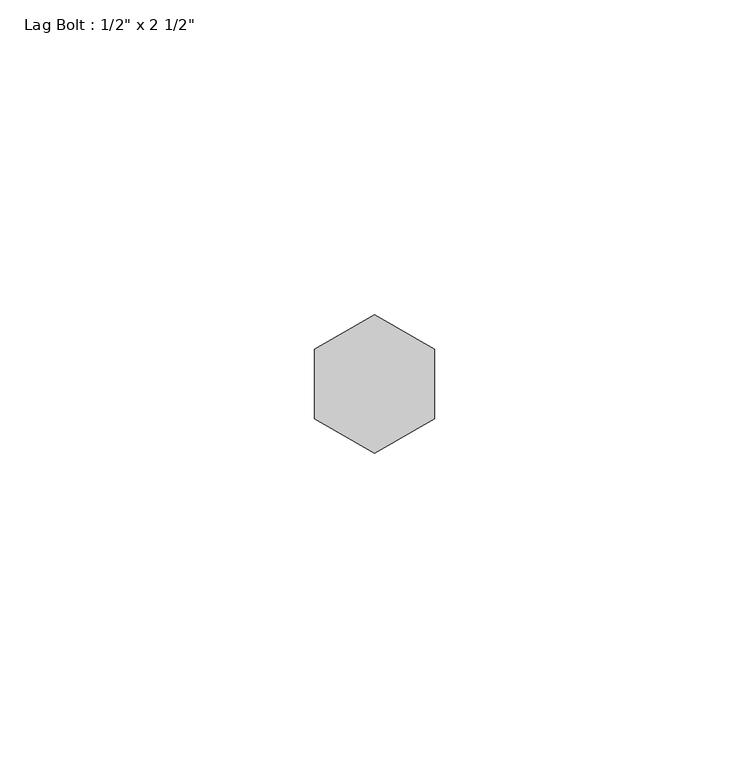
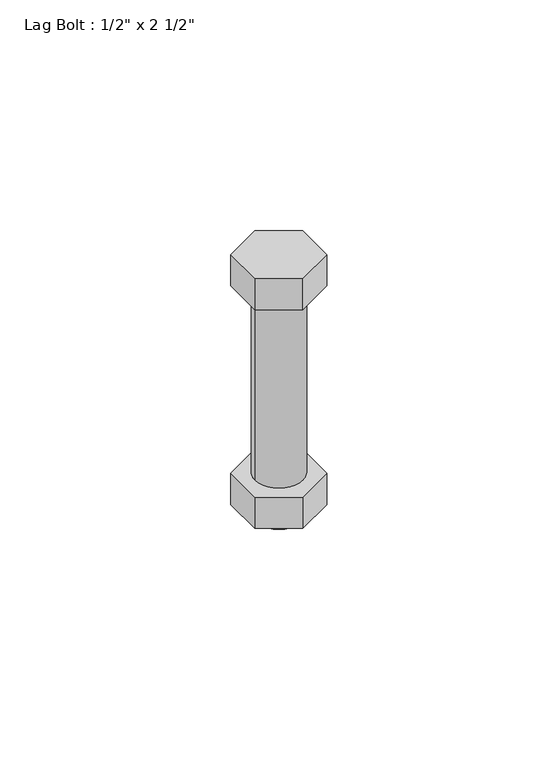
"""IFC4 building model written with IfcOpenShell, lengths in millimetres: proxy geometry."""

from ifc_helpers import new_model, si_unit, point, frame, origin, origin_with_axes, origin_2d, place, context, project, spatial, polyline, circle_curve, trimmed, segment, composite_curve, outline, extrude, source, transform, mapped, element, save


def proxy_eacf5a22(model_context):
    return source(origin(), model_context, "Body", "SweptSolid", [
        extrude(outline(polyline([(-9.525, 5.4992613), (0.0, 10.9985226), (9.525, 5.4992613), (9.525, -5.4992613), (0.0, -10.9985226), (-9.525, -5.4992613), (-9.525, 5.4992613)])), frame((0.0, 0.0, -61.0195313), z_axis=(0.0, 0.0, 1.0), x_axis=(1.0, 0.0, 0.0)), (0.0, 0.0, 1.0), 8.73125),
        extrude(outline(polyline([(-9.525, -5.4992613), (-9.525, 5.4992613), (0.0, 10.9985226), (9.525, 5.4992613), (9.525, -5.4992613), (0.0, -10.9985226), (-9.525, -5.4992613)])), origin_with_axes(), (0.0, 0.0, 1.0), 8.73125),
        extrude(outline(composite_curve([segment(trimmed(circle_curve(origin_2d(), 6.35), [point((-6.35, 0.0))], [point((6.35, 0.0))], False, "CARTESIAN"), True, "CONTINUOUS"), segment(trimmed(circle_curve(origin_2d(), 6.35), [point((6.35, 0.0))], [point((-6.35, 0.0))], False, "CARTESIAN"), True, "CONTINUOUS")], self_intersect=False)), frame((0.0, 0.0, -63.5), z_axis=(0.0, 0.0, 1.0), x_axis=(1.0, 0.0, 0.0)), (0.0, 0.0, 1.0), 63.5),
    ])


if __name__ == "__main__":
    model = new_model("IFC4")
    model_context = context("Model", 3, world=origin())
    ifc_project = project(units=[si_unit("LENGTHUNIT", "METRE", prefix="MILLI")], contexts=[model_context])
    site = spatial("IfcSite", under=ifc_project)
    building = spatial("IfcBuilding", under=site)
    placement = place(None, origin())
    proxy_shape = proxy_eacf5a22(model_context)
    element("IfcBuildingElementProxy", 1, Name="Lag Bolt : 1/2\" x 2 1/2\"", ObjectType="Lag Bolt : 1/2\" x 2 1/2\"", at=placement, inside=building, context=model_context, shape_type="MappedRepresentation", body=[
        mapped(proxy_shape, transform((0.0, 0.0, 0.0), x_axis=(1.0, 0.0, 0.0), y_axis=(0.0, 1.0, 0.0), z_axis=(0.0, 0.0, 1.0))),
    ])
    save(model, "model.ifc")

# Revit data of these elements
# Type "Lag Bolt : 1/2\" x 2 1/2\""
#   Thickness_of_Substrate [instance default] = 0' - 1"
#   Side = 0' - 0 111/256"
#   Radius = 0' - 0 1/4"
#   Length = 0' - 2 1/2"
#   Head Size = 0' - 0 3/4"
#   Head Radius = 0' - 0 3/8"
#   Head Height = 0' - 0 11/32"
#   Diameter = 0' - 0 1/2"
#   Default Elevation = 4' - 0"
#   Nut_Visibility [instance default] = yes
#   Bolt Material (Size) [instance default] = STRUCTURAL BOLTS (PAINT TO MATCH STEEL FINISH)
# Element 1 (IfcBuildingElementProxy, "Lag Bolt : 1/2\" x 2 1/2\"")
#   Thickness_of_Substrate = 0' - 2 15/256"
#   Bolt Material (Size) = THRU-BOLT OR LAG BOLT
#   Materials on its faces: "THRU-BOLT OR LAG BOLT"
# Materials
#   "STRUCTURAL BOLTS (PAINT TO MATCH STEEL FINISH)": class "Generic", colour RGB 120 120 120, transparency 0, Cost = 0
#   "THRU-BOLT OR LAG BOLT": class "Generic", colour RGB 120 120 120, transparency 0, Cost = 0
